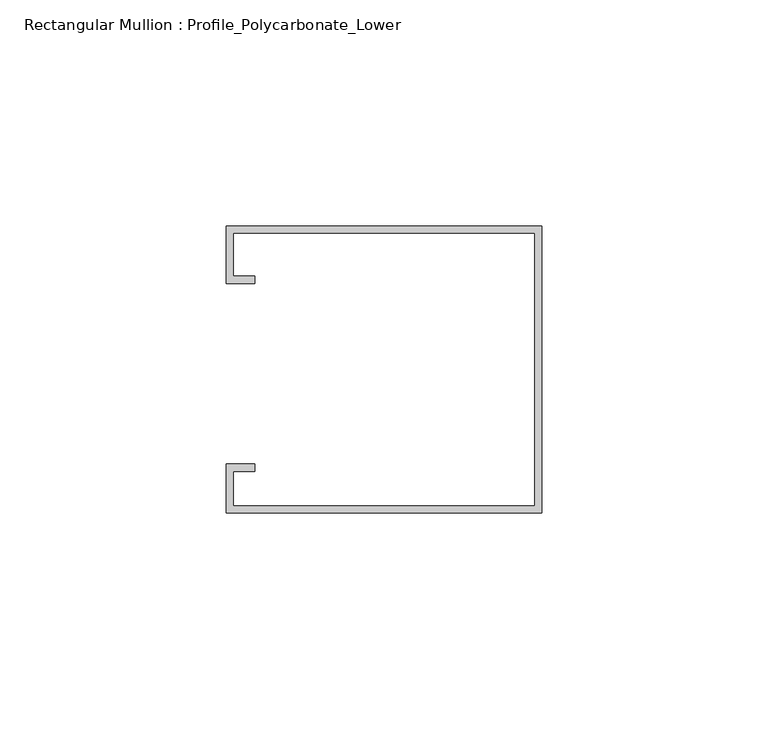
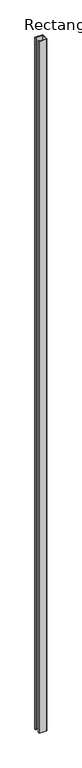
"""IFC4 building model written with IfcOpenShell, lengths in millimetres: member geometry, Rectangular Mullion : Profile_Polycarbonate_Lower."""

import ifcopenshell
import ifcopenshell.guid

model = None  # the IFC model being written
_history = None  # IfcOwnerHistory: only IFC2X3 demands one
_inside = {}  # id of a spatial element -> (the spatial element, [elements in it])
_under = {}  # id of a project, library or spatial element -> (it, [spatial elements below it])
_declared = {}  # id of a project -> (the project, [libraries it declares])
_typed = {}  # id of a type object -> (the type object, [elements of that type])
_made_of = {}  # id of a material, layer set ... -> (it, [elements and type objects made of it])


def new_model(schema):
    """Start an empty IFC model of exactly this schema.

    Asked for "IFC4X3", IfcOpenShell would pick the latest addendum, in which some entities
    have other attributes; the version numbers below select the first issue.
    IFC2X3 requires an IfcOwnerHistory on every rooted entity: one is made here for all.
    """
    global model, _history
    if schema == "IFC4X3":
        model = ifcopenshell.file(schema_version=(4, 3, 0, 0))
    else:
        model = ifcopenshell.file(schema=schema)
    _inside.clear()
    _under.clear()
    _declared.clear()
    _typed.clear()
    _made_of.clear()
    _history = None
    if model.schema == "IFC2X3":
        org = make("IfcOrganization", Name="unknown")
        user = make(
            "IfcPersonAndOrganization",
            ThePerson=make("IfcPerson", FamilyName="unknown"),
            TheOrganization=org,
        )
        app = make(
            "IfcApplication",
            ApplicationDeveloper=org,
            Version="unknown",
            ApplicationFullName="unknown",
            ApplicationIdentifier="unknown",
        )
        _history = make(
            "IfcOwnerHistory",
            OwningUser=user,
            OwningApplication=app,
            ChangeAction="ADDED",
            CreationDate=0,
        )
    return model


def make(cls, **values):
    """One entity of the class cls with the attributes given. An attribute that is None is left unset."""
    return model.create_entity(
        cls, **{name: value for name, value in values.items() if value is not None}
    )


def rooted(cls, **values):
    """An entity with a GlobalId (a new one), such as an element, a storey or a relation."""
    return make(cls, GlobalId=ifcopenshell.guid.new(), OwnerHistory=_history, **values)


def si_unit(unit_type, name, prefix=None):
    """IfcSIUnit, for example si_unit("LENGTHUNIT", "METRE", prefix="MILLI")."""
    return make("IfcSIUnit", UnitType=unit_type, Prefix=prefix, Name=name)


def assignment(units):
    """IfcUnitAssignment: the units of a project."""
    return None if units is None else make("IfcUnitAssignment", Units=units)


def point(xyz):
    """IfcCartesianPoint."""
    return None if xyz is None else make("IfcCartesianPoint", Coordinates=xyz)


def direction(xyz):
    """IfcDirection."""
    return None if xyz is None else make("IfcDirection", DirectionRatios=xyz)


def frame(location, z_axis=None, x_axis=None):
    """IfcAxis2Placement3D, a coordinate frame: its origin and axes. An axis left out is left unset."""
    return make(
        "IfcAxis2Placement3D",
        Location=point(location),
        Axis=direction(z_axis),
        RefDirection=direction(x_axis),
    )


def origin():
    """The frame at (0, 0, 0) with its axes left unset."""
    return frame((0.0, 0.0, 0.0))


def place(relative_to, where):
    """IfcLocalPlacement: puts the frame where relative to a parent placement (None: the world)."""
    return make(
        "IfcLocalPlacement", PlacementRelTo=relative_to, RelativePlacement=where
    )


def context(
    kind, dimensions, precision=None, world=None, true_north=None, identifier=None
):
    """IfcGeometricRepresentationContext, for example the 3D "Model" context."""
    return make(
        "IfcGeometricRepresentationContext",
        ContextIdentifier=identifier,
        ContextType=kind,
        CoordinateSpaceDimension=dimensions,
        Precision=precision,
        WorldCoordinateSystem=world,
        TrueNorth=true_north,
    )


def project(units=None, contexts=None):
    """IfcProject with its units and contexts."""
    return rooted(
        "IfcProject",
        Name="project",
        RepresentationContexts=contexts,
        UnitsInContext=assignment(units),
    )


def spatial(cls, under=None, at=None, **own):
    """A site, building, storey or space (cls), placed at a placement, below another one or the project."""
    s = rooted(cls, ObjectPlacement=at, **own)
    if under is not None:
        _under.setdefault(under.id(), (under, []))[1].append(s)
    return s


def polyline(points):
    """IfcPolyline through the points."""
    return make("IfcPolyline", Points=[point(p) for p in points])


def outline(outer, holes=None, kind="AREA"):
    """IfcArbitraryClosedProfileDef: a profile drawn as a closed curve; with holes, ...WithVoids."""
    if holes is None:
        return make("IfcArbitraryClosedProfileDef", ProfileType=kind, OuterCurve=outer)
    return make(
        "IfcArbitraryProfileDefWithVoids",
        ProfileType=kind,
        OuterCurve=outer,
        InnerCurves=holes,
    )


def extrude(swept, where, along, depth):
    """IfcExtrudedAreaSolid: the profile swept, set in the frame where, extruded along a direction by depth."""
    return make(
        "IfcExtrudedAreaSolid",
        SweptArea=swept,
        Position=where,
        ExtrudedDirection=direction(along),
        Depth=depth,
    )


def shape(context_of_items, identifier, shape_type, items):
    """IfcShapeRepresentation: the items that make up one representation, for example the "Body"."""
    return make(
        "IfcShapeRepresentation",
        ContextOfItems=context_of_items,
        RepresentationIdentifier=identifier,
        RepresentationType=shape_type,
        Items=items,
    )


def source(mapping_origin, context_of_items, identifier, shape_type, items):
    """IfcRepresentationMap: a shape defined once, which mapped items show again and again."""
    return make(
        "IfcRepresentationMap",
        MappingOrigin=mapping_origin,
        MappedRepresentation=shape(context_of_items, identifier, shape_type, items),
    )


def transform(
    local_origin,
    x_axis=None,
    y_axis=None,
    z_axis=None,
    scale=None,
    scale2=None,
    scale3=None,
    uniform=True,
):
    """IfcCartesianTransformationOperator3D, or its non-uniform kind. x_axis, y_axis, z_axis: its Axis1, 2, 3."""
    if uniform:
        return make(
            "IfcCartesianTransformationOperator3D",
            Axis1=direction(x_axis),
            Axis2=direction(y_axis),
            LocalOrigin=point(local_origin),
            Scale=scale,
            Axis3=direction(z_axis),
        )
    return make(
        "IfcCartesianTransformationOperator3DnonUniform",
        Axis1=direction(x_axis),
        Axis2=direction(y_axis),
        LocalOrigin=point(local_origin),
        Scale=scale,
        Axis3=direction(z_axis),
        Scale2=scale2,
        Scale3=scale3,
    )


def mapped(mapping_source, mapping_target):
    """IfcMappedItem: shows the shape of a source again, moved by a transform."""
    return make(
        "IfcMappedItem", MappingSource=mapping_source, MappingTarget=mapping_target
    )


def made_of(thing, what):
    """Note that an element or type object is made of a material, layer set ...; save() writes the relation."""
    if what is not None:
        _made_of.setdefault(what.id(), (what, []))[1].append(thing)
    return thing


def element(
    cls,
    number,
    at=None,
    inside=None,
    cuts=None,
    type_object=None,
    material=None,
    context=None,
    identifier="Body",
    shape_type=None,
    held_by="IfcProductDefinitionShape",
    body=None,
    shapes=None,
    **own,
):
    """One element of the class cls, such as IfcWall. Its Tag is "e" and its number.

    at: its placement. inside: the storey or other place that contains it. cuts: it is an
    opening in that element (IfcRelVoidsElement). A single representation is given by context,
    identifier, shape_type and body (its items); several are given by shapes. held_by: the class
    of the entity that holds the representations. save() writes the other relations.
    """
    e = rooted(cls, Tag="e%d" % number, ObjectPlacement=at, **own)
    if body is not None:
        shapes = [shape(context, identifier, shape_type, body)]
    if shapes is not None:
        e.Representation = make(held_by, Representations=shapes)
    if inside is not None:
        _inside.setdefault(inside.id(), (inside, []))[1].append(e)
    if cuts is not None:
        rooted(
            "IfcRelVoidsElement", RelatingBuildingElement=cuts, RelatedOpeningElement=e
        )
    if type_object is not None:
        _typed.setdefault(type_object.id(), (type_object, []))[1].append(e)
    return made_of(e, material)


def aggregate(whole, parts):
    """IfcRelAggregates: a whole, such as a stair, and the parts it consists of."""
    return rooted("IfcRelAggregates", RelatingObject=whole, RelatedObjects=parts)


def save(model, path):
    """Write the relations noted so far, then the file.

    IfcRelAggregates (storeys below a building ...), IfcRelContainedInSpatialStructure (elements
    in a storey), IfcRelDefinesByType, IfcRelAssociatesMaterial and IfcRelDeclares: one each for
    every whole, place, type object, material and project.
    """
    for whole, parts in _under.values():
        aggregate(whole, parts)
    for where, things in _inside.values():
        rooted(
            "IfcRelContainedInSpatialStructure",
            RelatedElements=things,
            RelatingStructure=where,
        )
    for kind, things in _typed.values():
        rooted("IfcRelDefinesByType", RelatedObjects=things, RelatingType=kind)
    for what, things in _made_of.values():
        rooted("IfcRelAssociatesMaterial", RelatedObjects=things, RelatingMaterial=what)
    for by, libraries in _declared.values():
        rooted("IfcRelDeclares", RelatingContext=by, RelatedDefinitions=libraries)
    model.write(path)


def rectangular_mullion_profile_polycarbonate_lower_94622d10(model_context):
    return source(origin(), model_context, "Body", "SweptSolid", [
        extrude(outline(polyline([(0.0, 32.7), (0.0, -30.8), (-69.85, -30.8), (-69.85, -20.0), (-63.5, -20.0), (-63.5, -21.5875), (-68.2625, -21.5875), (-68.2625, -29.2125), (-1.5875, -29.2125), (-1.5875, 31.1125), (-68.2625, 31.1125), (-68.2625, 21.5875), (-63.5, 21.5875), (-63.5, 20.0), (-69.85, 20.0), (-69.85, 32.7), (0.0, 32.7)])), frame((0.0, 0.0, -6550.025), z_axis=(0.0, 0.0, 1.0), x_axis=(1.0, 0.0, 0.0)), (0.0, 0.0, 1.0), 6550.025),
    ])


if __name__ == "__main__":
    model = new_model("IFC4")
    model_context = context("Model", 3, world=origin())
    ifc_project = project(units=[si_unit("LENGTHUNIT", "METRE", prefix="MILLI")], contexts=[model_context])
    site = spatial("IfcSite", under=ifc_project)
    building = spatial("IfcBuilding", under=site)
    placement = place(None, origin())
    rectangular_mullion_profile_polycarbonate_lower_shape = rectangular_mullion_profile_polycarbonate_lower_94622d10(model_context)
    element("IfcMember", 1, ObjectType="Rectangular Mullion : Profile_Polycarbonate_Lower", at=placement, inside=building, context=model_context, shape_type="MappedRepresentation", body=[
        mapped(rectangular_mullion_profile_polycarbonate_lower_shape, transform((0.0, 0.0, 0.0), x_axis=(1.0, 0.0, 0.0), y_axis=(0.0, 1.0, 0.0), z_axis=(0.0, 0.0, 1.0))),
    ])
    save(model, "model.ifc")

# Revit data of these elements
# Type "Rectangular Mullion : Profile_Polycarbonate_Lower"
#   built-in parameter 1007322 = 0.208333 (stored number, unit not read)
#   built-in parameter 1007321 = 0 (stored number, unit not read)
#   built-in parameter 1007320 = 0.00520833 (stored number, unit not read)
